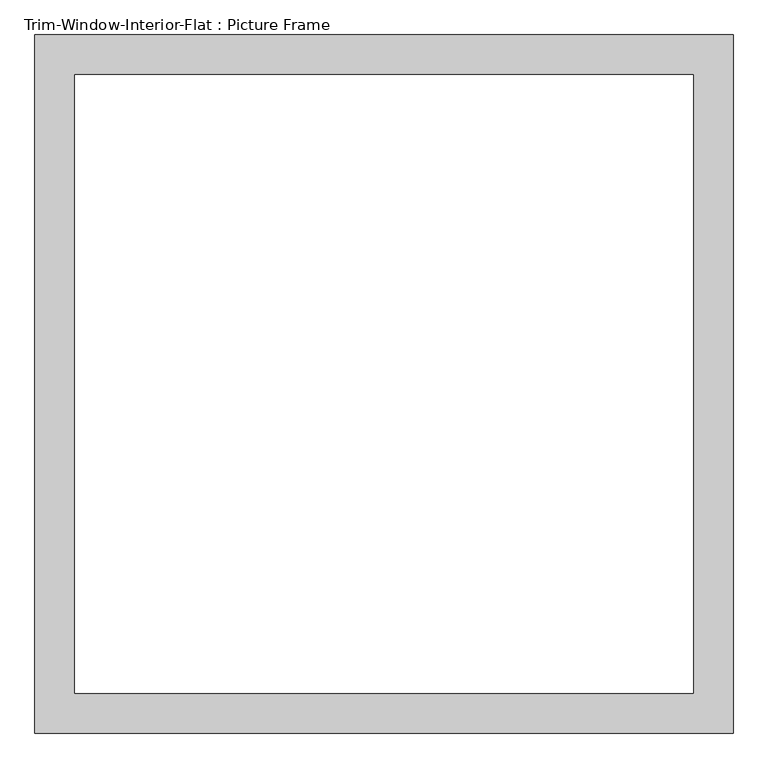
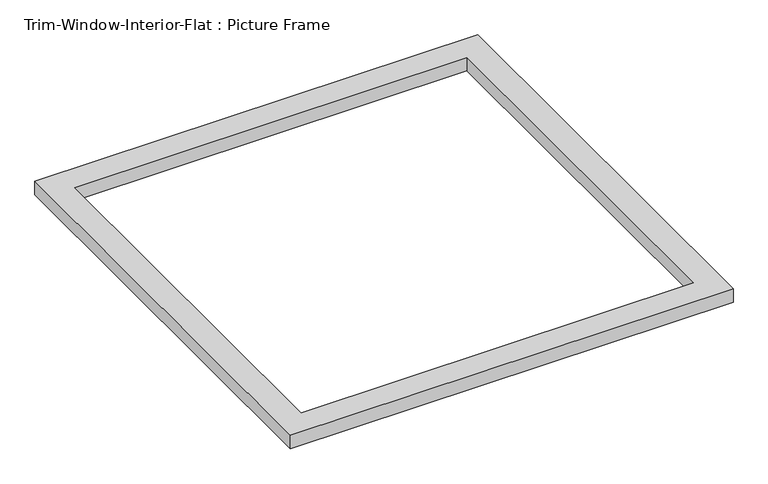
"""IFC4 building model written with IfcOpenShell, lengths in millimetres: proxy geometry, Trim-Window-Interior-Flat : Picture Frame."""

import ifcopenshell
import ifcopenshell.guid

model = None  # the IFC model being written
_history = None  # IfcOwnerHistory: only IFC2X3 demands one
_inside = {}  # id of a spatial element -> (the spatial element, [elements in it])
_under = {}  # id of a project, library or spatial element -> (it, [spatial elements below it])
_declared = {}  # id of a project -> (the project, [libraries it declares])
_typed = {}  # id of a type object -> (the type object, [elements of that type])
_made_of = {}  # id of a material, layer set ... -> (it, [elements and type objects made of it])


def new_model(schema):
    """Start an empty IFC model of exactly this schema.

    Asked for "IFC4X3", IfcOpenShell would pick the latest addendum, in which some entities
    have other attributes; the version numbers below select the first issue.
    IFC2X3 requires an IfcOwnerHistory on every rooted entity: one is made here for all.
    """
    global model, _history
    if schema == "IFC4X3":
        model = ifcopenshell.file(schema_version=(4, 3, 0, 0))
    else:
        model = ifcopenshell.file(schema=schema)
    _inside.clear()
    _under.clear()
    _declared.clear()
    _typed.clear()
    _made_of.clear()
    _history = None
    if model.schema == "IFC2X3":
        org = make("IfcOrganization", Name="unknown")
        user = make(
            "IfcPersonAndOrganization",
            ThePerson=make("IfcPerson", FamilyName="unknown"),
            TheOrganization=org,
        )
        app = make(
            "IfcApplication",
            ApplicationDeveloper=org,
            Version="unknown",
            ApplicationFullName="unknown",
            ApplicationIdentifier="unknown",
        )
        _history = make(
            "IfcOwnerHistory",
            OwningUser=user,
            OwningApplication=app,
            ChangeAction="ADDED",
            CreationDate=0,
        )
    return model


def make(cls, **values):
    """One entity of the class cls with the attributes given. An attribute that is None is left unset."""
    return model.create_entity(
        cls, **{name: value for name, value in values.items() if value is not None}
    )


def rooted(cls, **values):
    """An entity with a GlobalId (a new one), such as an element, a storey or a relation."""
    return make(cls, GlobalId=ifcopenshell.guid.new(), OwnerHistory=_history, **values)


def si_unit(unit_type, name, prefix=None):
    """IfcSIUnit, for example si_unit("LENGTHUNIT", "METRE", prefix="MILLI")."""
    return make("IfcSIUnit", UnitType=unit_type, Prefix=prefix, Name=name)


def assignment(units):
    """IfcUnitAssignment: the units of a project."""
    return None if units is None else make("IfcUnitAssignment", Units=units)


def point(xyz):
    """IfcCartesianPoint."""
    return None if xyz is None else make("IfcCartesianPoint", Coordinates=xyz)


def direction(xyz):
    """IfcDirection."""
    return None if xyz is None else make("IfcDirection", DirectionRatios=xyz)


def frame(location, z_axis=None, x_axis=None):
    """IfcAxis2Placement3D, a coordinate frame: its origin and axes. An axis left out is left unset."""
    return make(
        "IfcAxis2Placement3D",
        Location=point(location),
        Axis=direction(z_axis),
        RefDirection=direction(x_axis),
    )


def origin():
    """The frame at (0, 0, 0) with its axes left unset."""
    return frame((0.0, 0.0, 0.0))


def origin_with_axes():
    """The frame at (0, 0, 0) with the z axis (0, 0, 1) and the x axis (1, 0, 0) written out."""
    return frame((0.0, 0.0, 0.0), z_axis=(0.0, 0.0, 1.0), x_axis=(1.0, 0.0, 0.0))


def place(relative_to, where):
    """IfcLocalPlacement: puts the frame where relative to a parent placement (None: the world)."""
    return make(
        "IfcLocalPlacement", PlacementRelTo=relative_to, RelativePlacement=where
    )


def context(
    kind, dimensions, precision=None, world=None, true_north=None, identifier=None
):
    """IfcGeometricRepresentationContext, for example the 3D "Model" context."""
    return make(
        "IfcGeometricRepresentationContext",
        ContextIdentifier=identifier,
        ContextType=kind,
        CoordinateSpaceDimension=dimensions,
        Precision=precision,
        WorldCoordinateSystem=world,
        TrueNorth=true_north,
    )


def project(units=None, contexts=None):
    """IfcProject with its units and contexts."""
    return rooted(
        "IfcProject",
        Name="project",
        RepresentationContexts=contexts,
        UnitsInContext=assignment(units),
    )


def spatial(cls, under=None, at=None, **own):
    """A site, building, storey or space (cls), placed at a placement, below another one or the project."""
    s = rooted(cls, ObjectPlacement=at, **own)
    if under is not None:
        _under.setdefault(under.id(), (under, []))[1].append(s)
    return s


def polyline(points):
    """IfcPolyline through the points."""
    return make("IfcPolyline", Points=[point(p) for p in points])


def outline(outer, holes=None, kind="AREA"):
    """IfcArbitraryClosedProfileDef: a profile drawn as a closed curve; with holes, ...WithVoids."""
    if holes is None:
        return make("IfcArbitraryClosedProfileDef", ProfileType=kind, OuterCurve=outer)
    return make(
        "IfcArbitraryProfileDefWithVoids",
        ProfileType=kind,
        OuterCurve=outer,
        InnerCurves=holes,
    )


def extrude(swept, where, along, depth):
    """IfcExtrudedAreaSolid: the profile swept, set in the frame where, extruded along a direction by depth."""
    return make(
        "IfcExtrudedAreaSolid",
        SweptArea=swept,
        Position=where,
        ExtrudedDirection=direction(along),
        Depth=depth,
    )


def shape(context_of_items, identifier, shape_type, items):
    """IfcShapeRepresentation: the items that make up one representation, for example the "Body"."""
    return make(
        "IfcShapeRepresentation",
        ContextOfItems=context_of_items,
        RepresentationIdentifier=identifier,
        RepresentationType=shape_type,
        Items=items,
    )


def source(mapping_origin, context_of_items, identifier, shape_type, items):
    """IfcRepresentationMap: a shape defined once, which mapped items show again and again."""
    return make(
        "IfcRepresentationMap",
        MappingOrigin=mapping_origin,
        MappedRepresentation=shape(context_of_items, identifier, shape_type, items),
    )


def transform(
    local_origin,
    x_axis=None,
    y_axis=None,
    z_axis=None,
    scale=None,
    scale2=None,
    scale3=None,
    uniform=True,
):
    """IfcCartesianTransformationOperator3D, or its non-uniform kind. x_axis, y_axis, z_axis: its Axis1, 2, 3."""
    if uniform:
        return make(
            "IfcCartesianTransformationOperator3D",
            Axis1=direction(x_axis),
            Axis2=direction(y_axis),
            LocalOrigin=point(local_origin),
            Scale=scale,
            Axis3=direction(z_axis),
        )
    return make(
        "IfcCartesianTransformationOperator3DnonUniform",
        Axis1=direction(x_axis),
        Axis2=direction(y_axis),
        LocalOrigin=point(local_origin),
        Scale=scale,
        Axis3=direction(z_axis),
        Scale2=scale2,
        Scale3=scale3,
    )


def mapped(mapping_source, mapping_target):
    """IfcMappedItem: shows the shape of a source again, moved by a transform."""
    return make(
        "IfcMappedItem", MappingSource=mapping_source, MappingTarget=mapping_target
    )


def made_of(thing, what):
    """Note that an element or type object is made of a material, layer set ...; save() writes the relation."""
    if what is not None:
        _made_of.setdefault(what.id(), (what, []))[1].append(thing)
    return thing


def element(
    cls,
    number,
    at=None,
    inside=None,
    cuts=None,
    type_object=None,
    material=None,
    context=None,
    identifier="Body",
    shape_type=None,
    held_by="IfcProductDefinitionShape",
    body=None,
    shapes=None,
    **own,
):
    """One element of the class cls, such as IfcWall. Its Tag is "e" and its number.

    at: its placement. inside: the storey or other place that contains it. cuts: it is an
    opening in that element (IfcRelVoidsElement). A single representation is given by context,
    identifier, shape_type and body (its items); several are given by shapes. held_by: the class
    of the entity that holds the representations. save() writes the other relations.
    """
    e = rooted(cls, Tag="e%d" % number, ObjectPlacement=at, **own)
    if body is not None:
        shapes = [shape(context, identifier, shape_type, body)]
    if shapes is not None:
        e.Representation = make(held_by, Representations=shapes)
    if inside is not None:
        _inside.setdefault(inside.id(), (inside, []))[1].append(e)
    if cuts is not None:
        rooted(
            "IfcRelVoidsElement", RelatingBuildingElement=cuts, RelatedOpeningElement=e
        )
    if type_object is not None:
        _typed.setdefault(type_object.id(), (type_object, []))[1].append(e)
    return made_of(e, material)


def aggregate(whole, parts):
    """IfcRelAggregates: a whole, such as a stair, and the parts it consists of."""
    return rooted("IfcRelAggregates", RelatingObject=whole, RelatedObjects=parts)


def save(model, path):
    """Write the relations noted so far, then the file.

    IfcRelAggregates (storeys below a building ...), IfcRelContainedInSpatialStructure (elements
    in a storey), IfcRelDefinesByType, IfcRelAssociatesMaterial and IfcRelDeclares: one each for
    every whole, place, type object, material and project.
    """
    for whole, parts in _under.values():
        aggregate(whole, parts)
    for where, things in _inside.values():
        rooted(
            "IfcRelContainedInSpatialStructure",
            RelatedElements=things,
            RelatingStructure=where,
        )
    for kind, things in _typed.values():
        rooted("IfcRelDefinesByType", RelatedObjects=things, RelatingType=kind)
    for what, things in _made_of.values():
        rooted("IfcRelAssociatesMaterial", RelatedObjects=things, RelatingMaterial=what)
    for by, libraries in _declared.values():
        rooted("IfcRelDeclares", RelatingContext=by, RelatedDefinitions=libraries)
    model.write(path)


def trim_window_interior_flat_picture_frame_28d4e5dc(model_context):
    return source(origin(), model_context, "Body", "SweptSolid", [
        extrude(outline(polyline([(501.65, 44.45), (501.65, -958.85), (-501.65, -958.85), (-501.65, 44.45), (501.65, 44.45)]), holes=[polyline([(444.5, -12.7), (-444.5, -12.7), (-444.5, -901.7), (444.5, -901.7), (444.5, -12.7)])]), origin_with_axes(), (0.0, 0.0, 1.0), 31.75),
    ])


if __name__ == "__main__":
    model = new_model("IFC4")
    model_context = context("Model", 3, world=origin())
    ifc_project = project(units=[si_unit("LENGTHUNIT", "METRE", prefix="MILLI")], contexts=[model_context])
    site = spatial("IfcSite", under=ifc_project)
    building = spatial("IfcBuilding", under=site)
    placement = place(None, origin())
    trim_window_interior_flat_picture_frame_shape = trim_window_interior_flat_picture_frame_28d4e5dc(model_context)
    element("IfcBuildingElementProxy", 1, Name="Trim-Window-Interior-Flat : Picture Frame", ObjectType="Trim-Window-Interior-Flat : Picture Frame", at=placement, inside=building, context=model_context, shape_type="MappedRepresentation", body=[
        mapped(trim_window_interior_flat_picture_frame_shape, transform((0.0, 0.0, 0.0), x_axis=(1.0, 0.0, 0.0), y_axis=(0.0, 1.0, 0.0), z_axis=(0.0, 0.0, 1.0))),
    ])
    save(model, "model.ifc")

# Revit data of these elements
# Type "Trim-Window-Interior-Flat : Picture Frame"
#   Trim Thickness_Picture Frame = 0' - 1 1/4"
#   Trim Width = 0' - 2 1/4"
#   Trim Thickness_with Sill = 0' - 0 3/4"
#   Sill Thickness = 0' - 1 1/4"
#   Opening Width [instance default] = 2' - 0"
#   Opening Height [instance default] = 3' - 0"
#   Default Elevation = 4' - 0"
#   Sill = no
#   Picture Frame = yes
#   Trim Material [instance default] = none
# Element 1 (IfcBuildingElementProxy, "Trim-Window-Interior-Flat : Picture Frame")
#   Opening Width = 3' - 0"
#   Trim Material = Wood - Stained
#   Materials on its faces: "Wood - Stained"
# Materials
#   "Wood - Stained": class "Wood", colour RGB 224 178 126, transparency 0, Cost = 0
